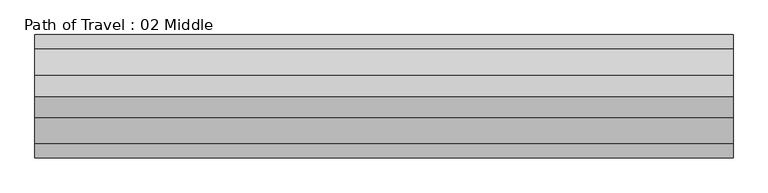
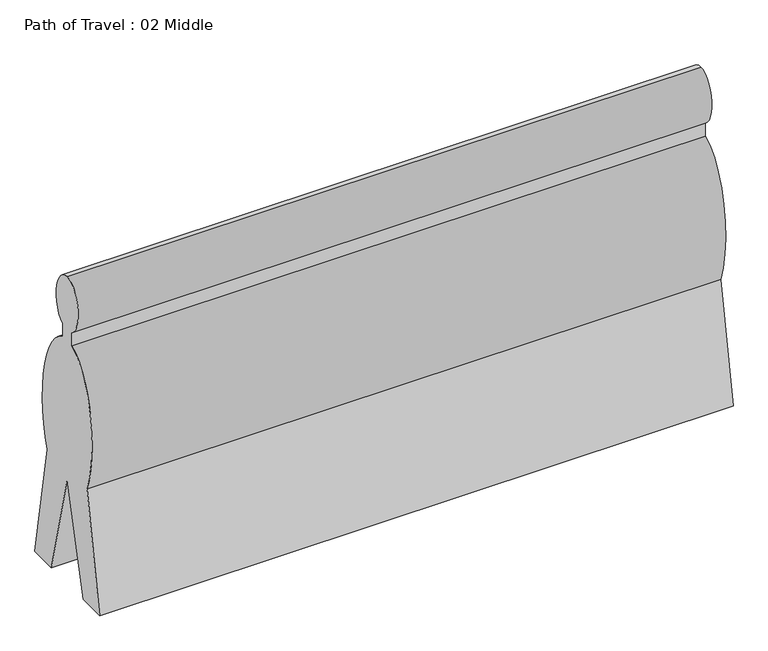
"""IFC4 building model written with IfcOpenShell, lengths in millimetres: proxy geometry, Path of Travel : 02 Middle."""

from ifc_helpers import new_model, si_unit, point, frame, origin, place, context, project, spatial, ellipse_curve, trimmed, source, transform, mapped, element, save
from ifc_brep_helpers import plane_surface, extruded_surface, advanced_brep


def path_of_travel_02_middle_87f58a54(model_context):
    return source(origin(), model_context, "Body", "AdvancedBrep", [
        advanced_brep(
        [(227.5554837, 0.0, 1727.2), (227.5554837, 42.9018657, 1436.6534209), (227.5554837, 42.9018657, 1363.4763406), (227.5554837, 184.1186263, 643.4144547), (227.5554837, 297.5699544, 0.0), (227.5554837, 145.6574193, 0.0), (227.5554837, 0.0, 584.2), (227.5554837, -145.6574193, 0.0), (227.5554837, -297.5699544, 0.0), (227.5554837, -184.1186263, 643.4144547), (227.5554837, -42.9018657, 1363.4763406), (227.5554837, -42.9018657, 1436.6534209), (3596.8100837, 0.0, 1727.2), (3596.8100837, -42.9018657, 1436.6534209), (3596.8100837, -42.9018657, 1363.4763406), (3596.8100837, -184.1186263, 643.4144547), (3596.8100837, -297.5699544, 0.0), (3596.8100837, -145.6574193, 0.0), (3596.8100837, 0.0, 584.2), (3596.8100837, 145.6574193, 0.0), (3596.8100837, 297.5699544, 0.0), (3596.8100837, 184.1186263, 643.4144547), (3596.8100837, 42.9018657, 1363.4763406), (3596.8100837, 42.9018657, 1436.6534209)],
        [
            (0, 1, ellipse_curve(frame((227.5554837, 0.0, 1574.8), z_axis=(-1.0, 0.0, 0.0), x_axis=(0.0, 0.0, 1.0)), 152.4, 101.6)),
            (1, 2),
            (2, 3, ellipse_curve(frame((227.5554837, 0.0, 914.4), z_axis=(-1.0, 0.0, 0.0), x_axis=(0.0, 0.0, -1.0)), 457.2, 228.6)),
            (3, 4),
            (4, 5),
            (5, 6),
            (6, 7),
            (7, 8),
            (8, 9),
            (9, 10, ellipse_curve(frame((227.5554837, 0.0, 914.4), z_axis=(-1.0, 0.0, 0.0), x_axis=(0.0, 0.0, -1.0)), 457.2, 228.6)),
            (10, 11),
            (11, 0, ellipse_curve(frame((227.5554837, 0.0, 1574.8), z_axis=(-1.0, 0.0, 0.0), x_axis=(0.0, 0.0, 1.0)), 152.4, 101.6)),
            (12, 13, ellipse_curve(frame((3596.8100837, 0.0, 1574.8), z_axis=(1.0, 0.0, 0.0), x_axis=(0.0, 0.0, 1.0)), 152.4, 101.6)),
            (13, 14),
            (14, 15, ellipse_curve(frame((3596.8100837, 0.0, 914.4), z_axis=(1.0, 0.0, 0.0), x_axis=(0.0, 0.0, -1.0)), 457.2, 228.6)),
            (15, 16),
            (16, 17),
            (17, 18),
            (18, 19),
            (19, 20),
            (20, 21),
            (21, 22, ellipse_curve(frame((3596.8100837, 0.0, 914.4), z_axis=(1.0, 0.0, 0.0), x_axis=(0.0, 0.0, -1.0)), 457.2, 228.6)),
            (22, 23),
            (23, 12, ellipse_curve(frame((3596.8100837, 0.0, 1574.8), z_axis=(1.0, 0.0, 0.0), x_axis=(0.0, 0.0, 1.0)), 152.4, 101.6)),
            (0, 12),
            (23, 1),
            (22, 2),
            (21, 3),
            (20, 4),
            (19, 5),
            (18, 6),
            (17, 7),
            (16, 8),
            (15, 9),
            (14, 10),
            (13, 11),
        ],
        [
            plane_surface(frame((227.5554837, 0.0, 0.0), z_axis=(-1.0, 0.0, 0.0), x_axis=(0.0, 0.0, 1.0))),
            plane_surface(frame((3596.8100837, 0.0, 0.0), z_axis=(1.0, 0.0, 0.0), x_axis=(0.0, 0.0, 1.0))),
            extruded_surface(trimmed(ellipse_curve(frame((3596.8100837, 0.0, 1574.8), z_axis=(-1.0, 0.0, 0.0), x_axis=(0.0, 0.0, 1.0)), 152.4, 101.6), [point((3596.8100837, 0.0, 1727.2))], [point((3596.8100837, 42.9018657, 1436.6534209))], True, "CARTESIAN"), (-3369.2546, 0.0, 0.0), 3369.2546),
            plane_surface(frame((227.5554837, 42.9018657, 1436.6534209), z_axis=(0.0, 1.0, 0.0), x_axis=(1.0, 0.0, 0.0))),
            extruded_surface(trimmed(ellipse_curve(frame((3596.8100837, 0.0, 914.4), z_axis=(-1.0, 0.0, 0.0), x_axis=(0.0, 0.0, -1.0)), 457.2, 228.6), [point((3596.8100837, 42.9018657, 1363.4763406))], [point((3596.8100837, 184.1186263, 643.4144547))], True, "CARTESIAN"), (-3369.2546, 0.0, 0.0), 3369.2546),
            plane_surface(frame((227.5554837, 184.1186263, 643.4144547), z_axis=(0.0, 0.9848077530122078, 0.17364817766693205), x_axis=(1.0, 0.0, 0.0))),
            plane_surface(frame((227.5554837, 297.5699544, 0.0), z_axis=(0.0, 0.0, -1.0), x_axis=(1.0, 0.0, 0.0))),
            plane_surface(frame((227.5554837, 145.6574193, 0.0), z_axis=(0.0, -0.9702957262760199, -0.2419218955995739), x_axis=(1.0, 0.0, 0.0))),
            plane_surface(frame((227.5554837, 0.0, 584.2), z_axis=(0.0, 0.9702957262759961, -0.24192189559966923), x_axis=(1.0, 0.0, 0.0))),
            plane_surface(frame((227.5554837, -145.6574193, 0.0), z_axis=(0.0, 0.0, -1.0), x_axis=(1.0, 0.0, 0.0))),
            plane_surface(frame((227.5554837, -297.5699544, 0.0), z_axis=(0.0, -0.984807753012208, 0.17364817766693066), x_axis=(1.0, 0.0, 0.0))),
            extruded_surface(trimmed(ellipse_curve(frame((3596.8100837, 0.0, 914.4), z_axis=(-1.0, 0.0, 0.0), x_axis=(0.0, 0.0, -1.0)), 457.2, 228.6), [point((3596.8100837, -184.1186263, 643.4144547))], [point((3596.8100837, -42.9018657, 1363.4763406))], True, "CARTESIAN"), (-3369.2546, 0.0, 0.0), 3369.2546),
            plane_surface(frame((227.5554837, -42.9018657, 1363.4763406), z_axis=(0.0, -1.0, 0.0), x_axis=(1.0, 0.0, 0.0))),
            extruded_surface(trimmed(ellipse_curve(frame((3596.8100837, 0.0, 1574.8), z_axis=(-1.0, 0.0, 0.0), x_axis=(0.0, 0.0, 1.0)), 152.4, 101.6), [point((3596.8100837, -42.9018657, 1436.6534209))], [point((3596.8100837, 0.0, 1727.2))], True, "CARTESIAN"), (-3369.2546, 0.0, 0.0), 3369.2546),
        ],
        [
            (0, [[1, 2, 3, 4, 5, 6, 7, 8, 9, 10, 11, 12]]),
            (1, [[13, 14, 15, 16, 17, 18, 19, 20, 21, 22, 23, 24]]),
            (2, [[-1, 25, -24, 26]]),
            (3, [[-2, -26, -23, 27]]),
            (4, [[-3, -27, -22, 28]]),
            (5, [[-4, -28, -21, 29]]),
            (6, [[-5, -29, -20, 30]]),
            (7, [[-6, -30, -19, 31]]),
            (8, [[-7, -31, -18, 32]]),
            (9, [[-8, -32, -17, 33]]),
            (10, [[-9, -33, -16, 34]]),
            (11, [[-10, -34, -15, 35]]),
            (12, [[-11, -35, -14, 36]]),
            (13, [[-12, -36, -13, -25]]),
        ],
    ),
    ])


if __name__ == "__main__":
    model = new_model("IFC4")
    model_context = context("Model", 3, world=origin())
    ifc_project = project(units=[si_unit("LENGTHUNIT", "METRE", prefix="MILLI")], contexts=[model_context])
    site = spatial("IfcSite", under=ifc_project)
    building = spatial("IfcBuilding", under=site)
    placement = place(None, origin())
    path_of_travel_02_middle_shape = path_of_travel_02_middle_87f58a54(model_context)
    element("IfcBuildingElementProxy", 1, Name="Path of Travel : 02 Middle", ObjectType="Path of Travel : 02 Middle", at=placement, inside=building, context=model_context, shape_type="MappedRepresentation", body=[
        mapped(path_of_travel_02_middle_shape, transform((0.0, 0.0, 0.0), x_axis=(1.0, 0.0, 0.0), y_axis=(0.0, 1.0, 0.0), z_axis=(0.0, 0.0, 1.0))),
    ])
    save(model, "model.ifc")

# Revit data of these elements
# Type "Path of Travel : 02 Middle"
#   Path of Egress [instance default] = 4' - 0"
#   built-in parameter 1001306 [instance default] = 4 (stored number, unit not read)
#   Dot at Start = no
#   Arrow in Middle = yes
#   Arrow at End = no
#   Egress Path = none
# Element 1 (IfcBuildingElementProxy, "Path of Travel : 02 Middle")
#   Path of Egress = 11' - 0.64782"
#   built-in parameter 1001306 = 11.054 (stored number, unit not read)
#   Materials on its faces: "Egress Path Solid"
# Materials
#   "Egress Path Solid": class "Unassigned", colour RGB 255 128 64, transparency 0.75, Comments = "Rendering appearance not upgraded "
